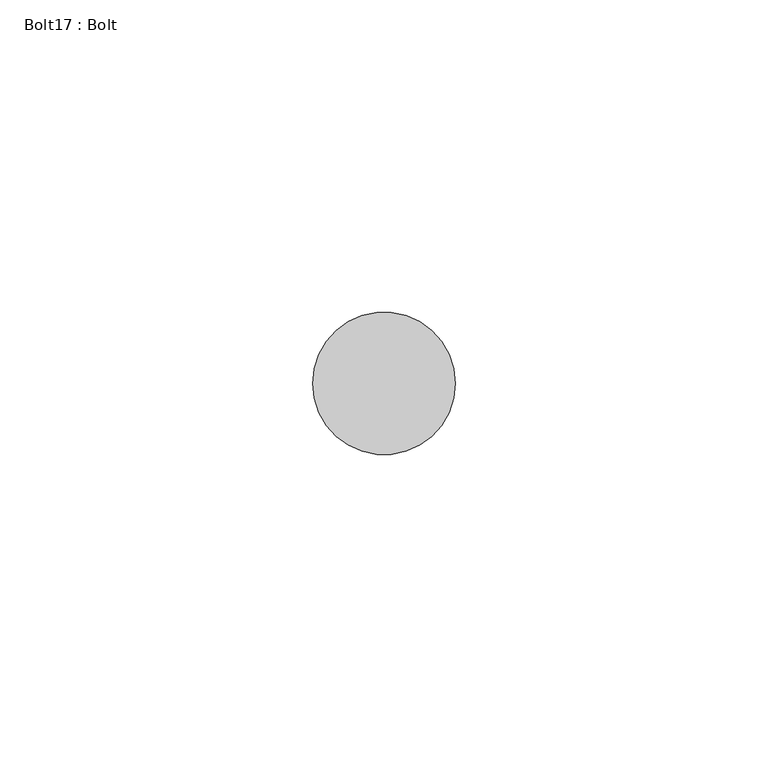
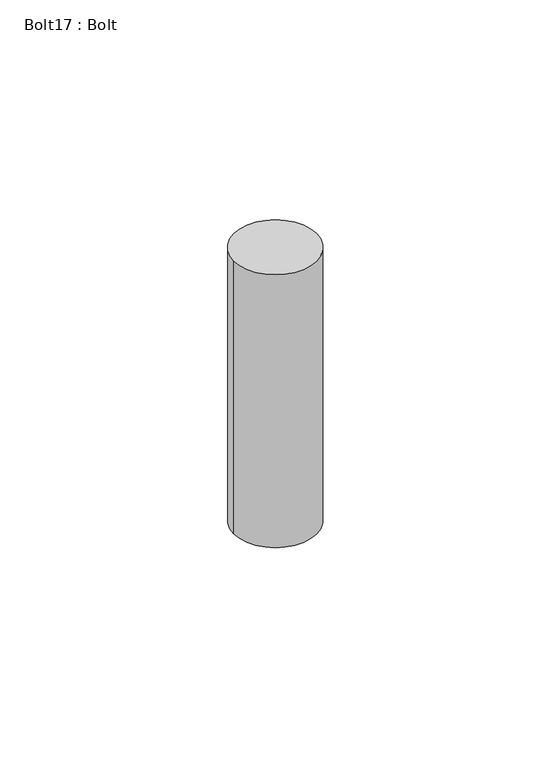
"""IFC4 building model written with IfcOpenShell, lengths in millimetres: proxy geometry, Bolt17 : Bolt."""

from ifc_helpers import new_model, si_unit, point, frame, frame_2d, origin, place, context, project, spatial, circle_curve, trimmed, segment, composite_curve, outline, extrude, source, transform, mapped, element, save


def bolt17_bolt_1f82a6c6(model_context):
    return source(origin(), model_context, "Body", "SweptSolid", [
        extrude(outline(composite_curve([segment(trimmed(circle_curve(frame_2d((7251.9702148, -1781.8449707)), 11.4045168), [point((7240.565698, -1781.8449707))], [point((7263.3747317, -1781.8449707))], False, "CARTESIAN"), True, "CONTINUOUS"), segment(trimmed(circle_curve(frame_2d((7251.9702148, -1781.8449707)), 11.4045168), [point((7263.3747317, -1781.8449707))], [point((7240.565698, -1781.8449707))], False, "CARTESIAN"), True, "CONTINUOUS")], self_intersect=False)), frame((0.0, 0.0, 40049.196), z_axis=(0.0, 0.0, 1.0), x_axis=(1.0, 0.0, 0.0)), (0.0, 0.0, 1.0), 79.375),
    ])


if __name__ == "__main__":
    model = new_model("IFC4")
    model_context = context("Model", 3, world=origin())
    ifc_project = project(units=[si_unit("LENGTHUNIT", "METRE", prefix="MILLI")], contexts=[model_context])
    site = spatial("IfcSite", under=ifc_project)
    building = spatial("IfcBuilding", under=site)
    placement = place(None, origin())
    bolt17_bolt_shape = bolt17_bolt_1f82a6c6(model_context)
    element("IfcBuildingElementProxy", 1, Name="Bolt17 : Bolt", ObjectType="Bolt17 : Bolt", at=placement, inside=building, context=model_context, shape_type="MappedRepresentation", body=[
        mapped(bolt17_bolt_shape, transform((0.0, 0.0, 0.0), x_axis=(1.0, 0.0, 0.0), y_axis=(0.0, 1.0, 0.0), z_axis=(0.0, 0.0, 1.0))),
    ])
    save(model, "model.ifc")

# Revit data of these elements
# Type "Bolt17 : Bolt"
#   NameOverride = "Bolt"
# Element 1 (IfcBuildingElementProxy, "Bolt17 : Bolt")
#   Materials on its faces: "BOLTS CONCEALED BY FLOOR FINISH"
# Materials
#   "BOLTS CONCEALED BY FLOOR FINISH": class "Unassigned", colour RGB 128 128 128, transparency 0
